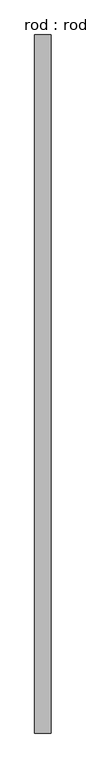
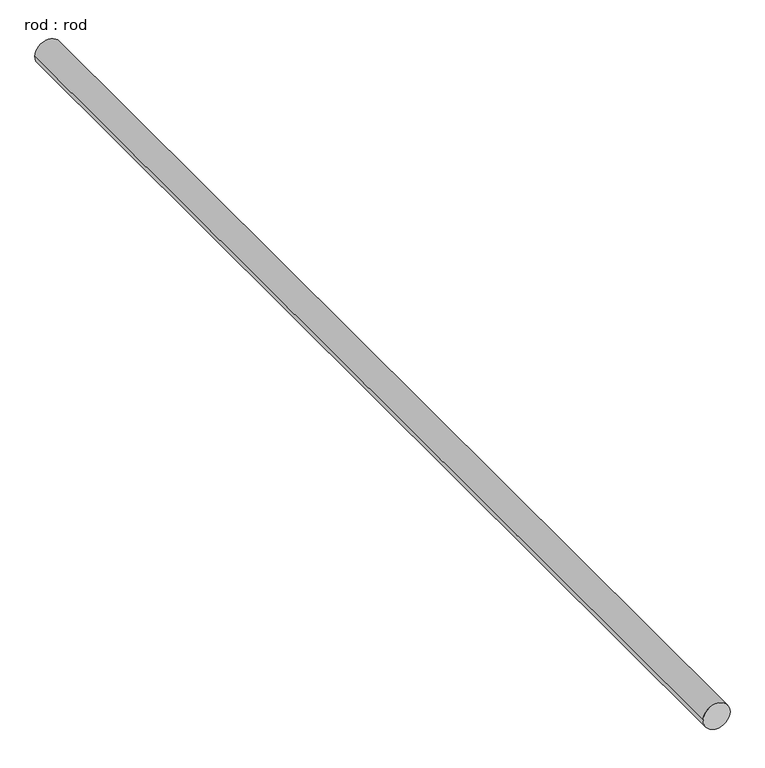
"""IFC4 building model written with IfcOpenShell, lengths in millimetres: proxy geometry, rod : rod."""

from ifc_helpers import new_model, si_unit, point, frame, frame_2d, origin, place, context, project, spatial, circle_curve, trimmed, segment, composite_curve, outline, extrude, source, transform, mapped, element, save


def rod_rod_4531df86(model_context):
    return source(origin(), model_context, "Body", "SweptSolid", [
        extrude(outline(composite_curve([segment(trimmed(circle_curve(frame_2d((0.0108462, 0.0)), 200.0), [point((0.0108462, 200.0))], [point((0.0108462, -200.0))], False, "CARTESIAN"), True, "CONTINUOUS"), segment(trimmed(circle_curve(frame_2d((0.0108462, 0.0)), 200.0), [point((0.0108462, -200.0))], [point((0.0108462, 200.0))], False, "CARTESIAN"), True, "CONTINUOUS")], self_intersect=False)), frame((0.0, -4532.2713847, 0.0), z_axis=(0.0, 1.0, 0.0), x_axis=(0.0, 0.0, 1.0)), (0.0, 0.0, 1.0), 17250.0),
    ])


if __name__ == "__main__":
    model = new_model("IFC4")
    model_context = context("Model", 3, world=origin())
    ifc_project = project(units=[si_unit("LENGTHUNIT", "METRE", prefix="MILLI")], contexts=[model_context])
    site = spatial("IfcSite", under=ifc_project)
    building = spatial("IfcBuilding", under=site)
    placement = place(None, origin())
    rod_rod_shape = rod_rod_4531df86(model_context)
    element("IfcBuildingElementProxy", 1, Name="rod : rod", ObjectType="rod : rod", at=placement, inside=building, context=model_context, shape_type="MappedRepresentation", body=[
        mapped(rod_rod_shape, transform((0.0, 0.0, 0.0), x_axis=(1.0, 0.0, 0.0), y_axis=(0.0, 1.0, 0.0), z_axis=(0.0, 0.0, 1.0))),
    ])
    save(model, "model.ifc")

# Revit data of these elements
# Type "rod : rod"
#   Default Elevation = 0
